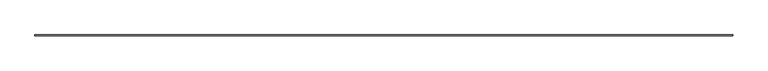
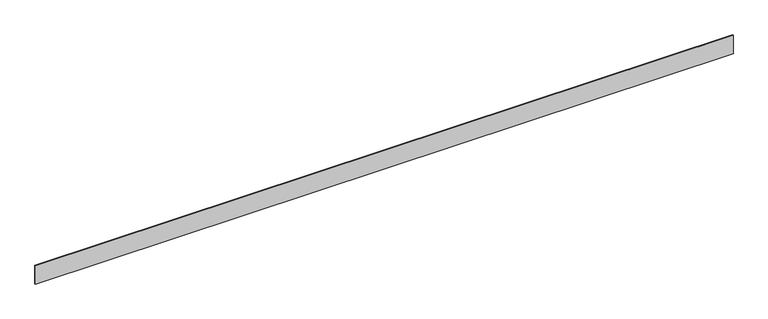
"""IFC4 building model written with IfcOpenShell, lengths in millimetres: proxy geometry, Generic Models 7:Generic Models 1:6:Generic Models 1:6 : Generic Models 7:Generic Models 1:337419:13 : Generic Models 7:Generic Models 1:6:Generic Models 1:6 : Generic Models 7:Generic Models 1:337419:312901."""

from ifc_helpers import new_model, si_unit, frame, origin, place, context, project, spatial, polyline, outline, extrude, source, transform, mapped, element, save


def generic_models_761c7fec(model_context):
    return source(origin(), model_context, "Body", "SweptSolid", [
        extrude(outline(polyline([(602310.5867239, -579089.5913841), (602310.5867239, -579140.3913841), (557809.7867239, -579140.3913841), (557809.7867239, -579089.5913841), (602310.5867239, -579089.5913841)])), frame((0.0, 0.0, -1222.375), z_axis=(0.0, 0.0, 1.0), x_axis=(1.0, 0.0, 0.0)), (0.0, 0.0, 1.0), 1223.0401798),
    ])


if __name__ == "__main__":
    model = new_model("IFC4")
    model_context = context("Model", 3, world=origin())
    ifc_project = project(units=[si_unit("LENGTHUNIT", "METRE", prefix="MILLI")], contexts=[model_context])
    site = spatial("IfcSite", under=ifc_project)
    building = spatial("IfcBuilding", under=site)
    placement = place(None, origin())
    generic_models_shape = generic_models_761c7fec(model_context)
    element("IfcBuildingElementProxy", 1, Name="Generic Models 7:Generic Models 1:6:Generic Models 1:6 : Generic Models 7:Generic Models 1:337419:13 : Generic Models 7:Generic Models 1:6:Generic Models 1:6 : Generic Models 7:Generic Models 1:337419:312901", ObjectType="Generic Models 7:Generic Models 1:6:Generic Models 1:6 : Generic Models 7:Generic Models 1:337419:13 : Generic Models 7:Generic Models 1:6:Generic Models 1:6 : Generic Models 7:Generic Models 1:337419:312901", at=placement, inside=building, context=model_context, shape_type="MappedRepresentation", body=[
        mapped(generic_models_shape, transform((0.0, 0.0, 0.0), x_axis=(1.0, 0.0, 0.0), y_axis=(0.0, 1.0, 0.0), z_axis=(0.0, 0.0, 1.0))),
    ])
    save(model, "model.ifc")

# Revit data of these elements
# Type "Generic Models 7:Generic Models 1:6:Generic Models 1:6 : Generic Models 7:Generic Models 1:337419:13 : Generic Models 7:Generic Models 1:6:Generic Models 1:6 : Generic Models 7:Generic Models 1:337419:312901"
#   NameOverride = "Generic Models 7:Generic Models 1:6:Generic Models 1:6 : Generic Models 7:Generic Models 1:337419:312901"
#   ObjectTypeOverride = "Generic Models 1:6 : Generic Models 7:Generic Models 1:337419"
#   Reference = "Generic Models 1"
#   Tag = "312901"
# Element 1 (IfcBuildingElementProxy, "Generic Models 7:Generic Models 1:6:Generic Models 1:6 : Generic Models 7:Generic Models 1:337419:13 : Generic Models 7:Generic Models 1:6:Generic Models 1:6 : Generic Models 7:Generic Models 1:337419:312901")
#   Materials on its faces: "EXTRUDED POLYSTYRENE (XPS) RIGID FOAM INSULATION (FOAMULAR® 250 OR SIMILAR)"
# Materials
#   "EXTRUDED POLYSTYRENE (XPS) RIGID FOAM INSULATION (FOAMULAR® 250 OR SIMILAR)": class "Unassigned", colour RGB 247 185 194, transparency 0, Cost = 0
